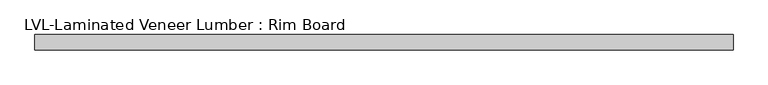
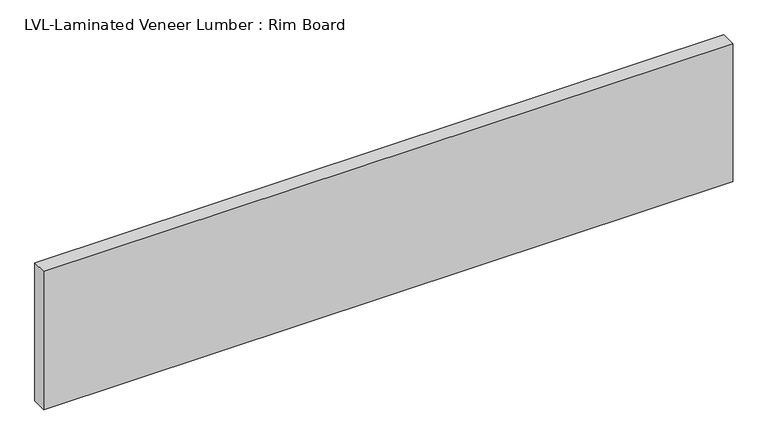
"""IFC4 building model written with IfcOpenShell, lengths in millimetres: beam geometry, LVL-Laminated Veneer Lumber : Rim Board."""

from ifc_helpers import new_model, si_unit, frame, origin, place, context, project, spatial, polyline, outline, extrude, source, transform, mapped, element, save


def lvl_laminated_veneer_lumber_rim_board_1d56c707(model_context):
    return source(origin(), model_context, "Body", "SweptSolid", [
        extrude(outline(polyline([(727.075, 15.875), (727.075, -15.875), (-695.325, -15.875), (-695.325, 15.875), (727.075, 15.875)])), frame((0.0, 0.0, -150.8125), z_axis=(0.0, 0.0, 1.0), x_axis=(1.0, 0.0, 0.0)), (0.0, 0.0, 1.0), 301.625),
    ])


if __name__ == "__main__":
    model = new_model("IFC4")
    model_context = context("Model", 3, world=origin())
    ifc_project = project(units=[si_unit("LENGTHUNIT", "METRE", prefix="MILLI")], contexts=[model_context])
    site = spatial("IfcSite", under=ifc_project)
    building = spatial("IfcBuilding", under=site)
    placement = place(None, origin())
    lvl_laminated_veneer_lumber_rim_board_shape = lvl_laminated_veneer_lumber_rim_board_1d56c707(model_context)
    element("IfcBeam", 1, ObjectType="LVL-Laminated Veneer Lumber : Rim Board", at=placement, inside=building, context=model_context, shape_type="MappedRepresentation", body=[
        mapped(lvl_laminated_veneer_lumber_rim_board_shape, transform((0.0, 0.0, 0.0), x_axis=(1.0, 0.0, 0.0), y_axis=(0.0, 1.0, 0.0), z_axis=(0.0, 0.0, 1.0))),
    ])
    save(model, "model.ifc")

# Revit data of these elements
# Type "LVL-Laminated Veneer Lumber : Rim Board"
#   Assembly Code = "B10"
#   Cost = 4.6
#   Length [instance default] = 5' - 0"
#   b = 0' - 1 1/4"
#   d = 0' - 11 7/8"
#   Structural Material [instance default] = Softwood, Lumber
# Element 1 (IfcBeam, "LVL-Laminated Veneer Lumber : Rim Board")
#   Structural Material = Douglas Fir #2
#   Materials on its faces: "Douglas Fir #2"
# Materials
#   "Softwood, Lumber": class "Wood", colour RGB 223 192 134, transparency 0, Description = "Pinus Echinata", Cost = 0
#   "Douglas Fir #2": class "Wood", colour RGB 223 192 134, transparency 0, Description = "Pinus Echinata", Cost = 0
